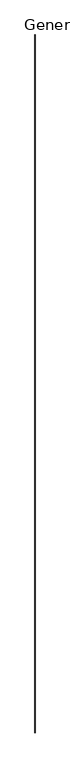
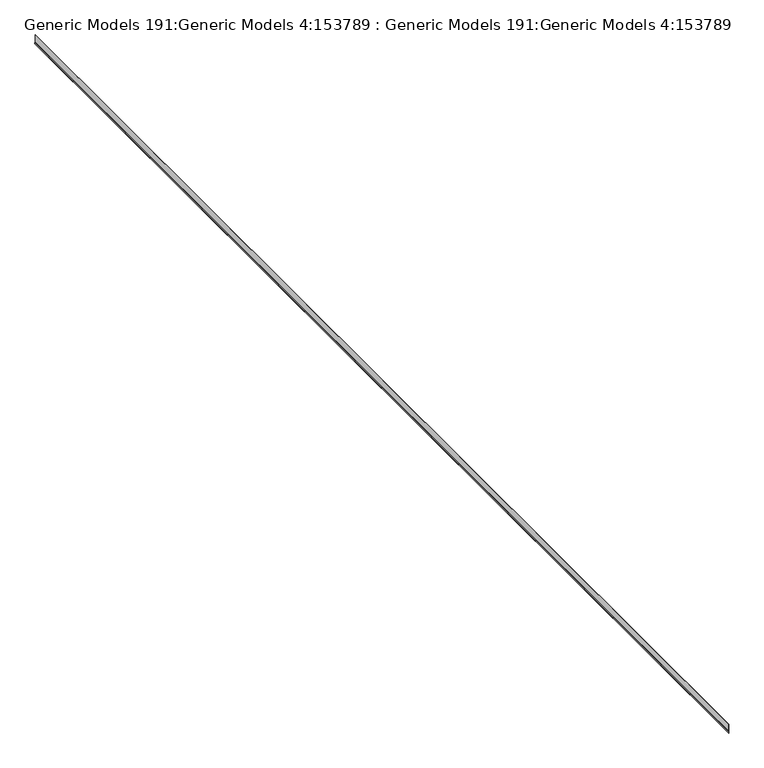
"""IFC4 building model written with IfcOpenShell, lengths in millimetres: proxy geometry, Generic Models 191:Generic Models 4:153789 : Generic Models 191:Generic Models 4:153789."""

from ifc_helpers import new_model, si_unit, frame, origin, place, context, project, spatial, polyline, outline, extrude, source, transform, mapped, element, save


def generic_models_191_generic_models_4_153789_generic_models_a5bee7c5(model_context):
    return source(origin(), model_context, "Body", "SweptSolid", [
        extrude(outline(polyline([(5948.7697814, -5377.0533304), (5959.8635277, -5373.015537), (6079.1052418, -5373.015537), (6079.1052418, -5373.809287), (5960.0034872, -5373.809287), (5948.909741, -5377.8470804), (5933.8559784, -5377.8470804), (5933.8559784, -5377.0533304), (5948.7697814, -5377.0533304)])), frame((0.0, -6674.7974793, 0.0), z_axis=(0.0, 1.0, 0.0), x_axis=(0.0, 0.0, 1.0)), (0.0, 0.0, 1.0), 18643.6),
    ])


if __name__ == "__main__":
    model = new_model("IFC4")
    model_context = context("Model", 3, world=origin())
    ifc_project = project(units=[si_unit("LENGTHUNIT", "METRE", prefix="MILLI")], contexts=[model_context])
    site = spatial("IfcSite", under=ifc_project)
    building = spatial("IfcBuilding", under=site)
    placement = place(None, origin())
    generic_models_191_generic_models_4_153789_generic_models_shape = generic_models_191_generic_models_4_153789_generic_models_a5bee7c5(model_context)
    element("IfcBuildingElementProxy", 1, Name="Generic Models 191:Generic Models 4:153789 : Generic Models 191:Generic Models 4:153789", ObjectType="Generic Models 191:Generic Models 4:153789 : Generic Models 191:Generic Models 4:153789", at=placement, inside=building, context=model_context, shape_type="MappedRepresentation", body=[
        mapped(generic_models_191_generic_models_4_153789_generic_models_shape, transform((0.0, 0.0, 0.0), x_axis=(1.0, 0.0, 0.0), y_axis=(0.0, 1.0, 0.0), z_axis=(0.0, 0.0, 1.0))),
    ])
    save(model, "model.ifc")

# Revit data of these elements
# Type "Generic Models 191:Generic Models 4:153789 : Generic Models 191:Generic Models 4:153789"
#   NameOverride = "Generic Models 191:Generic Models 4:153789"
#   ObjectTypeOverride = "Generic Models 191:Generic Models 4"
#   Reference = "Generic Models 4"
#   Category = "Generic Models"
#   Tag = "153789"
# Element 1 (IfcBuildingElementProxy, "Generic Models 191:Generic Models 4:153789 : Generic Models 191:Generic Models 4:153789")
#   Materials on its faces: "_(2) LAYERS NO. 30 ASTM D226 ASPHALT SATURATED ORGANIC FELT 997"
# Materials
#   "_(2) LAYERS NO. 30 ASTM D226 ASPHALT SATURATED ORGANIC FELT 997": class "Unassigned", colour RGB 67 154 161, transparency 0
